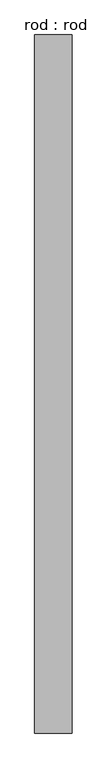
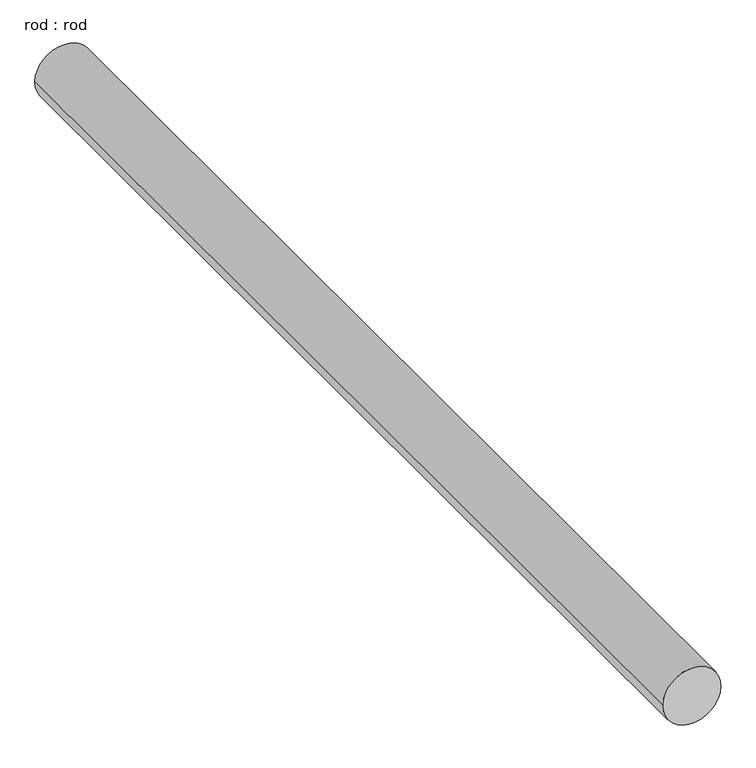
"""IFC4 building model written with IfcOpenShell, lengths in millimetres: proxy geometry, rod : rod."""

from ifc_helpers import new_model, si_unit, point, frame, frame_2d, origin, place, context, project, spatial, circle_curve, trimmed, segment, composite_curve, outline, extrude, source, transform, mapped, element, save


def rod_rod_b4072f8a(model_context):
    return source(origin(), model_context, "Body", "SweptSolid", [
        extrude(outline(composite_curve([segment(trimmed(circle_curve(frame_2d((0.0108462, 0.0)), 200.0), [point((0.0108462, 200.0))], [point((0.0108462, -200.0))], False, "CARTESIAN"), True, "CONTINUOUS"), segment(trimmed(circle_curve(frame_2d((0.0108462, 0.0)), 200.0), [point((0.0108462, -200.0))], [point((0.0108462, 200.0))], False, "CARTESIAN"), True, "CONTINUOUS")], self_intersect=False)), frame((0.0, 375.4419285, 0.0), z_axis=(0.0, 1.0, 0.0), x_axis=(0.0, 0.0, 1.0)), (0.0, 0.0, 1.0), 7434.5733738),
    ])


if __name__ == "__main__":
    model = new_model("IFC4")
    model_context = context("Model", 3, world=origin())
    ifc_project = project(units=[si_unit("LENGTHUNIT", "METRE", prefix="MILLI")], contexts=[model_context])
    site = spatial("IfcSite", under=ifc_project)
    building = spatial("IfcBuilding", under=site)
    placement = place(None, origin())
    rod_rod_shape = rod_rod_b4072f8a(model_context)
    element("IfcBuildingElementProxy", 1, Name="rod : rod", ObjectType="rod : rod", at=placement, inside=building, context=model_context, shape_type="MappedRepresentation", body=[
        mapped(rod_rod_shape, transform((0.0, 0.0, 0.0), x_axis=(1.0, 0.0, 0.0), y_axis=(0.0, 1.0, 0.0), z_axis=(0.0, 0.0, 1.0))),
    ])
    save(model, "model.ifc")

# Revit data of these elements
# Type "rod : rod"
#   Default Elevation = 0
